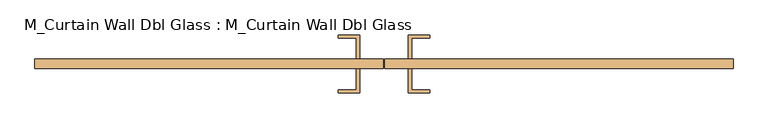
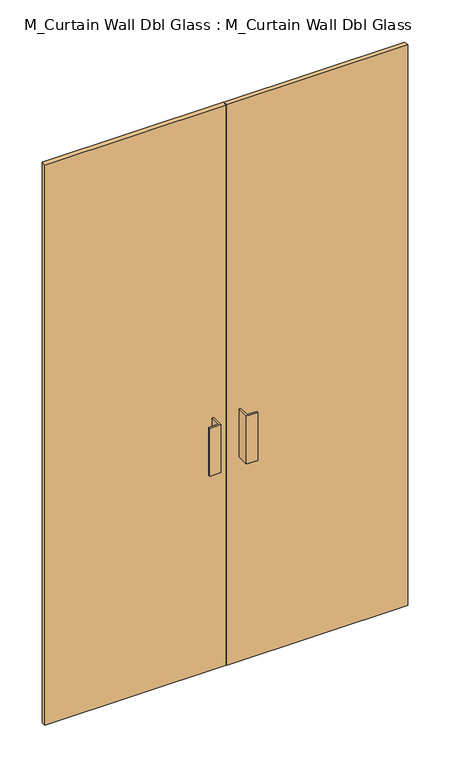
"""IFC4 building model written with IfcOpenShell, lengths in millimetres: door geometry, M_Curtain Wall Dbl Glass : M_Curtain Wall Dbl Glass."""

from ifc_helpers import new_model, si_unit, frame, origin, origin_with_axes, place, context, project, spatial, polyline, outline, extrude, source, transform, mapped, element, save


def m_curtain_wall_dbl_glass_m_curtain_wall_dbl_glass_6be05337(model_context):
    return source(origin(), model_context, "Body", "SweptSolid", [
        extrude(outline(polyline([(-1.5875, 30.95), (-725.0, 30.95), (-725.0, 50.0), (-1.5875, 50.0), (-1.5875, 30.95)])), origin_with_axes(), (0.0, 0.0, 1.0), 2370.0),
        extrude(outline(polyline([(725.0, 30.95), (1.5875, 30.95), (1.5875, 50.0), (725.0, 50.0), (725.0, 30.95)])), origin_with_axes(), (0.0, 0.0, 1.0), 2370.0),
        extrude(outline(polyline([(-50.8, 100.8), (-50.8, 50.0), (-57.15, 50.0), (-57.15, 94.45), (-95.25, 94.45), (-95.25, 100.8), (-50.8, 100.8)])), frame((0.0, 0.0, 863.6), z_axis=(0.0, 0.0, 1.0), x_axis=(1.0, 0.0, 0.0)), (0.0, 0.0, 1.0), 203.2),
        extrude(outline(polyline([(50.8, 100.8), (95.25, 100.8), (95.25, 94.45), (57.15, 94.45), (57.15, 50.0), (50.8, 50.0), (50.8, 100.8)])), frame((0.0, 0.0, 863.6), z_axis=(0.0, 0.0, 1.0), x_axis=(1.0, 0.0, 0.0)), (0.0, 0.0, 1.0), 203.2),
        extrude(outline(polyline([(-50.8, -19.85), (-95.25, -19.85), (-95.25, -13.5), (-57.15, -13.5), (-57.15, 30.95), (-50.8, 30.95), (-50.8, -19.85)])), frame((0.0, 0.0, 863.6), z_axis=(0.0, 0.0, 1.0), x_axis=(1.0, 0.0, 0.0)), (0.0, 0.0, 1.0), 203.2),
        extrude(outline(polyline([(50.8, -19.85), (50.8, 30.95), (57.15, 30.95), (57.15, -13.5), (95.25, -13.5), (95.25, -19.85), (50.8, -19.85)])), frame((0.0, 0.0, 863.6), z_axis=(0.0, 0.0, 1.0), x_axis=(1.0, 0.0, 0.0)), (0.0, 0.0, 1.0), 203.2),
    ])


if __name__ == "__main__":
    model = new_model("IFC4")
    model_context = context("Model", 3, world=origin())
    ifc_project = project(units=[si_unit("LENGTHUNIT", "METRE", prefix="MILLI")], contexts=[model_context])
    site = spatial("IfcSite", under=ifc_project)
    building = spatial("IfcBuilding", under=site)
    placement = place(None, origin())
    m_curtain_wall_dbl_glass_m_curtain_wall_dbl_glass_shape = m_curtain_wall_dbl_glass_m_curtain_wall_dbl_glass_6be05337(model_context)
    element("IfcDoor", 1, ObjectType="M_Curtain Wall Dbl Glass : M_Curtain Wall Dbl Glass", at=placement, inside=building, context=model_context, shape_type="MappedRepresentation", body=[
        mapped(m_curtain_wall_dbl_glass_m_curtain_wall_dbl_glass_shape, transform((0.0, 0.0, 0.0), x_axis=(1.0, 0.0, 0.0), y_axis=(0.0, 1.0, 0.0), z_axis=(0.0, 0.0, 1.0))),
    ])
    save(model, "model.ifc")

# Revit data of these elements
# Type "M_Curtain Wall Dbl Glass : M_Curtain Wall Dbl Glass"
#   Model = "12345678"
#   Manufacturer = "Dublin Doors"
#   Description = "Double Glass Door"
#   Type Mark = "41"
#   COBie.Type.CreatedBy = "design@eagle.com"
#   COBie.Type.CreatedOn = "2016-09-13T05:47:35"
#   COBie.Type.Name = "Doors_M_Curtain Wall Dbl Glass_M_Curtain Wall Dbl Glass"
#   COBie.Type.Category = "23-30 10 00 : Doors"
#   COBie.Type.Description = "Double Glass Door"
#   COBie.Type.Manufacturer = "Dublin Doors"
#   COBie.Type.ModelNumber = "12345678"
#   Construction Type Id = "GSP4R"
#   Analytic Construction = "1/8 in Pilkington single glazing"
#   COBie.Type.ReplacementCost = 0
#   Visual Light Transmittance = 0.9
#   Solar Heat Gain Coefficient = 0.78
#   Offset = 50 mm
#   Heat Transfer Coefficient (U) = 3.6886 W/(m²·K)
#   COBie.Type = yes
#   Function = 1
#   Glazing Material = Glass
# Element 1 (IfcDoor, "M_Curtain Wall Dbl Glass : M_Curtain Wall Dbl Glass")
#   Materials on its faces: "Aluminum", "Glass"
# Materials
#   "Glass": class "Glass", colour RGB 0 128 192, transparency 0.75, Description = "Soda Lime Glass", Cost = 0
#   "Aluminum": class "Metal", colour RGB 247 247 247, transparency 0, Description = "Aluminum 6061", Cost = 0
